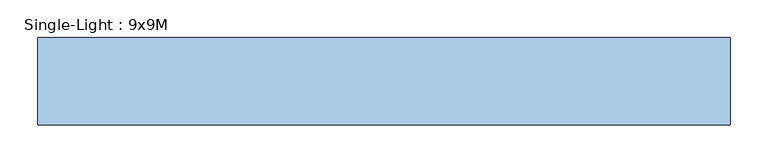
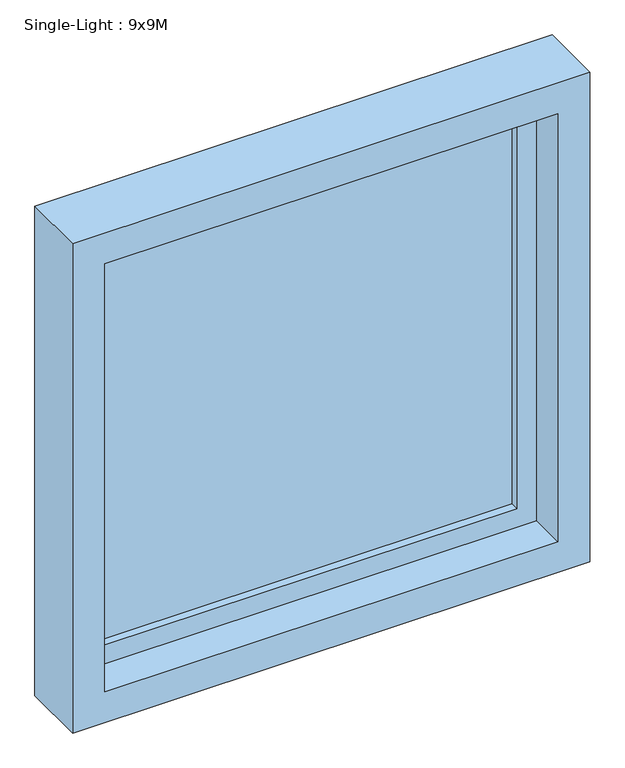
"""IFC4 building model written with IfcOpenShell, lengths in millimetres: window geometry, Single-Light : 9x9M."""

import ifcopenshell
import ifcopenshell.guid

model = None  # the IFC model being written
_history = None  # IfcOwnerHistory: only IFC2X3 demands one
_inside = {}  # id of a spatial element -> (the spatial element, [elements in it])
_under = {}  # id of a project, library or spatial element -> (it, [spatial elements below it])
_declared = {}  # id of a project -> (the project, [libraries it declares])
_typed = {}  # id of a type object -> (the type object, [elements of that type])
_made_of = {}  # id of a material, layer set ... -> (it, [elements and type objects made of it])


def new_model(schema):
    """Start an empty IFC model of exactly this schema.

    Asked for "IFC4X3", IfcOpenShell would pick the latest addendum, in which some entities
    have other attributes; the version numbers below select the first issue.
    IFC2X3 requires an IfcOwnerHistory on every rooted entity: one is made here for all.
    """
    global model, _history
    if schema == "IFC4X3":
        model = ifcopenshell.file(schema_version=(4, 3, 0, 0))
    else:
        model = ifcopenshell.file(schema=schema)
    _inside.clear()
    _under.clear()
    _declared.clear()
    _typed.clear()
    _made_of.clear()
    _history = None
    if model.schema == "IFC2X3":
        org = make("IfcOrganization", Name="unknown")
        user = make(
            "IfcPersonAndOrganization",
            ThePerson=make("IfcPerson", FamilyName="unknown"),
            TheOrganization=org,
        )
        app = make(
            "IfcApplication",
            ApplicationDeveloper=org,
            Version="unknown",
            ApplicationFullName="unknown",
            ApplicationIdentifier="unknown",
        )
        _history = make(
            "IfcOwnerHistory",
            OwningUser=user,
            OwningApplication=app,
            ChangeAction="ADDED",
            CreationDate=0,
        )
    return model


def make(cls, **values):
    """One entity of the class cls with the attributes given. An attribute that is None is left unset."""
    return model.create_entity(
        cls, **{name: value for name, value in values.items() if value is not None}
    )


def rooted(cls, **values):
    """An entity with a GlobalId (a new one), such as an element, a storey or a relation."""
    return make(cls, GlobalId=ifcopenshell.guid.new(), OwnerHistory=_history, **values)


def si_unit(unit_type, name, prefix=None):
    """IfcSIUnit, for example si_unit("LENGTHUNIT", "METRE", prefix="MILLI")."""
    return make("IfcSIUnit", UnitType=unit_type, Prefix=prefix, Name=name)


def assignment(units):
    """IfcUnitAssignment: the units of a project."""
    return None if units is None else make("IfcUnitAssignment", Units=units)


def point(xyz):
    """IfcCartesianPoint."""
    return None if xyz is None else make("IfcCartesianPoint", Coordinates=xyz)


def direction(xyz):
    """IfcDirection."""
    return None if xyz is None else make("IfcDirection", DirectionRatios=xyz)


def frame(location, z_axis=None, x_axis=None):
    """IfcAxis2Placement3D, a coordinate frame: its origin and axes. An axis left out is left unset."""
    return make(
        "IfcAxis2Placement3D",
        Location=point(location),
        Axis=direction(z_axis),
        RefDirection=direction(x_axis),
    )


def origin():
    """The frame at (0, 0, 0) with its axes left unset."""
    return frame((0.0, 0.0, 0.0))


def place(relative_to, where):
    """IfcLocalPlacement: puts the frame where relative to a parent placement (None: the world)."""
    return make(
        "IfcLocalPlacement", PlacementRelTo=relative_to, RelativePlacement=where
    )


def context(
    kind, dimensions, precision=None, world=None, true_north=None, identifier=None
):
    """IfcGeometricRepresentationContext, for example the 3D "Model" context."""
    return make(
        "IfcGeometricRepresentationContext",
        ContextIdentifier=identifier,
        ContextType=kind,
        CoordinateSpaceDimension=dimensions,
        Precision=precision,
        WorldCoordinateSystem=world,
        TrueNorth=true_north,
    )


def project(units=None, contexts=None):
    """IfcProject with its units and contexts."""
    return rooted(
        "IfcProject",
        Name="project",
        RepresentationContexts=contexts,
        UnitsInContext=assignment(units),
    )


def spatial(cls, under=None, at=None, **own):
    """A site, building, storey or space (cls), placed at a placement, below another one or the project."""
    s = rooted(cls, ObjectPlacement=at, **own)
    if under is not None:
        _under.setdefault(under.id(), (under, []))[1].append(s)
    return s


def polyline(points):
    """IfcPolyline through the points."""
    return make("IfcPolyline", Points=[point(p) for p in points])


def outline(outer, holes=None, kind="AREA"):
    """IfcArbitraryClosedProfileDef: a profile drawn as a closed curve; with holes, ...WithVoids."""
    if holes is None:
        return make("IfcArbitraryClosedProfileDef", ProfileType=kind, OuterCurve=outer)
    return make(
        "IfcArbitraryProfileDefWithVoids",
        ProfileType=kind,
        OuterCurve=outer,
        InnerCurves=holes,
    )


def extrude(swept, where, along, depth):
    """IfcExtrudedAreaSolid: the profile swept, set in the frame where, extruded along a direction by depth."""
    return make(
        "IfcExtrudedAreaSolid",
        SweptArea=swept,
        Position=where,
        ExtrudedDirection=direction(along),
        Depth=depth,
    )


def faces_of(points, faces, orient=None, outer=None):
    """IfcFace entities. A face is a list of loops; a loop is a list of indices into points, from 0.

    orient and outer hold one flag for each loop. By default every Orientation is true, the
    first loop of a face is its IfcFaceOuterBound and the others are IfcFaceBound.
    """
    made = []
    for i, loops in enumerate(faces):
        bounds = []
        for j, loop in enumerate(loops):
            is_outer = j == 0 if outer is None else outer[i][j]
            bounds.append(
                make(
                    "IfcFaceOuterBound" if is_outer else "IfcFaceBound",
                    Bound=make("IfcPolyLoop", Polygon=[points[k] for k in loop]),
                    Orientation=True if orient is None else orient[i][j],
                )
            )
        made.append(make("IfcFace", Bounds=bounds))
    return made


def faceted_brep(points, faces, orient=None, outer=None, voids=None):
    """IfcFacetedBrep: a solid bounded by flat faces; with voids (closed shells), ...WithVoids."""
    shared = [point(p) for p in points]
    hull = make("IfcClosedShell", CfsFaces=faces_of(shared, faces, orient, outer))
    if voids is None:
        return make("IfcFacetedBrep", Outer=hull)
    return make(
        "IfcFacetedBrepWithVoids",
        Outer=hull,
        Voids=[
            make(cls, CfsFaces=faces_of(shared, fs, o, b)) for cls, fs, o, b in voids
        ],
    )


def shape(context_of_items, identifier, shape_type, items):
    """IfcShapeRepresentation: the items that make up one representation, for example the "Body"."""
    return make(
        "IfcShapeRepresentation",
        ContextOfItems=context_of_items,
        RepresentationIdentifier=identifier,
        RepresentationType=shape_type,
        Items=items,
    )


def source(mapping_origin, context_of_items, identifier, shape_type, items):
    """IfcRepresentationMap: a shape defined once, which mapped items show again and again."""
    return make(
        "IfcRepresentationMap",
        MappingOrigin=mapping_origin,
        MappedRepresentation=shape(context_of_items, identifier, shape_type, items),
    )


def transform(
    local_origin,
    x_axis=None,
    y_axis=None,
    z_axis=None,
    scale=None,
    scale2=None,
    scale3=None,
    uniform=True,
):
    """IfcCartesianTransformationOperator3D, or its non-uniform kind. x_axis, y_axis, z_axis: its Axis1, 2, 3."""
    if uniform:
        return make(
            "IfcCartesianTransformationOperator3D",
            Axis1=direction(x_axis),
            Axis2=direction(y_axis),
            LocalOrigin=point(local_origin),
            Scale=scale,
            Axis3=direction(z_axis),
        )
    return make(
        "IfcCartesianTransformationOperator3DnonUniform",
        Axis1=direction(x_axis),
        Axis2=direction(y_axis),
        LocalOrigin=point(local_origin),
        Scale=scale,
        Axis3=direction(z_axis),
        Scale2=scale2,
        Scale3=scale3,
    )


def mapped(mapping_source, mapping_target):
    """IfcMappedItem: shows the shape of a source again, moved by a transform."""
    return make(
        "IfcMappedItem", MappingSource=mapping_source, MappingTarget=mapping_target
    )


def made_of(thing, what):
    """Note that an element or type object is made of a material, layer set ...; save() writes the relation."""
    if what is not None:
        _made_of.setdefault(what.id(), (what, []))[1].append(thing)
    return thing


def element(
    cls,
    number,
    at=None,
    inside=None,
    cuts=None,
    type_object=None,
    material=None,
    context=None,
    identifier="Body",
    shape_type=None,
    held_by="IfcProductDefinitionShape",
    body=None,
    shapes=None,
    **own,
):
    """One element of the class cls, such as IfcWall. Its Tag is "e" and its number.

    at: its placement. inside: the storey or other place that contains it. cuts: it is an
    opening in that element (IfcRelVoidsElement). A single representation is given by context,
    identifier, shape_type and body (its items); several are given by shapes. held_by: the class
    of the entity that holds the representations. save() writes the other relations.
    """
    e = rooted(cls, Tag="e%d" % number, ObjectPlacement=at, **own)
    if body is not None:
        shapes = [shape(context, identifier, shape_type, body)]
    if shapes is not None:
        e.Representation = make(held_by, Representations=shapes)
    if inside is not None:
        _inside.setdefault(inside.id(), (inside, []))[1].append(e)
    if cuts is not None:
        rooted(
            "IfcRelVoidsElement", RelatingBuildingElement=cuts, RelatedOpeningElement=e
        )
    if type_object is not None:
        _typed.setdefault(type_object.id(), (type_object, []))[1].append(e)
    return made_of(e, material)


def aggregate(whole, parts):
    """IfcRelAggregates: a whole, such as a stair, and the parts it consists of."""
    return rooted("IfcRelAggregates", RelatingObject=whole, RelatedObjects=parts)


def save(model, path):
    """Write the relations noted so far, then the file.

    IfcRelAggregates (storeys below a building ...), IfcRelContainedInSpatialStructure (elements
    in a storey), IfcRelDefinesByType, IfcRelAssociatesMaterial and IfcRelDeclares: one each for
    every whole, place, type object, material and project.
    """
    for whole, parts in _under.values():
        aggregate(whole, parts)
    for where, things in _inside.values():
        rooted(
            "IfcRelContainedInSpatialStructure",
            RelatedElements=things,
            RelatingStructure=where,
        )
    for kind, things in _typed.values():
        rooted("IfcRelDefinesByType", RelatedObjects=things, RelatingType=kind)
    for what, things in _made_of.values():
        rooted("IfcRelAssociatesMaterial", RelatedObjects=things, RelatingMaterial=what)
    for by, libraries in _declared.values():
        rooted("IfcRelDeclares", RelatingContext=by, RelatedDefinitions=libraries)
    model.write(path)


def single_light_9x9m_9d4aa27d(model_context):
    return source(origin(), model_context, "Body", "SolidModel", [
        extrude(outline(polyline([(1670.0, -414.0), (842.0, -414.0), (842.0, 414.0), (1670.0, 414.0), (1670.0, -414.0)]), holes=[polyline([(1620.0, 364.0), (892.0, 364.0), (892.0, -364.0), (1620.0, -364.0), (1620.0, 364.0)])]), frame((0.0, 134.0, 0.0), z_axis=(0.0, 1.0, 0.0), x_axis=(0.0, 0.0, 1.0)), (0.0, 0.0, 1.0), 50.0),
        faceted_brep([(-456.0, 69.0, 800.0), (-456.0, 184.0, 800.0), (456.0, 184.0, 800.0), (456.0, 69.0, 800.0), (456.0, 184.0, 1712.0), (456.0, 69.0, 1712.0), (-456.0, 184.0, 1712.0), (414.0, 184.0, 1670.0), (-414.0, 184.0, 1670.0), (-414.0, 184.0, 842.0), (414.0, 184.0, 842.0), (-456.0, 69.0, 1712.0), (399.0, 69.0, 857.0), (-399.0, 69.0, 857.0), (-399.0, 69.0, 1655.0), (399.0, 69.0, 1655.0), (-399.0, 134.0, 857.0), (399.0, 134.0, 857.0), (399.0, 134.0, 1655.0), (414.0, 134.0, 842.0), (-414.0, 134.0, 842.0), (-414.0, 134.0, 1670.0), (414.0, 134.0, 1670.0), (-399.0, 134.0, 1655.0)], [[[0, 1, 2, 3]], [[3, 2, 4, 5]], [[2, 1, 6, 4], [7, 8, 9, 10]], [[5, 11, 0, 3], [12, 13, 14, 15]], [[16, 13, 12, 17]], [[17, 12, 15, 18]], [[19, 20, 21, 22], [18, 23, 16, 17]], [[9, 20, 19, 10]], [[10, 19, 22, 7]], [[11, 6, 1, 0]], [[23, 14, 13, 16]], [[8, 21, 20, 9]], [[5, 4, 6, 11]], [[18, 15, 14, 23]], [[7, 22, 21, 8]]]),
        extrude(outline(polyline([(-364.0, 170.0), (364.0, 170.0), (364.0, 148.0), (-364.0, 148.0), (-364.0, 170.0)])), frame((0.0, 0.0, 892.0), z_axis=(0.0, 0.0, 1.0), x_axis=(1.0, 0.0, 0.0)), (0.0, 0.0, 1.0), 728.0),
    ])


if __name__ == "__main__":
    model = new_model("IFC4")
    model_context = context("Model", 3, world=origin())
    ifc_project = project(units=[si_unit("LENGTHUNIT", "METRE", prefix="MILLI")], contexts=[model_context])
    site = spatial("IfcSite", under=ifc_project)
    building = spatial("IfcBuilding", under=site)
    placement = place(None, origin())
    single_light_9x9m_shape = single_light_9x9m_9d4aa27d(model_context)
    element("IfcWindow", 1, ObjectType="Single-Light : 9x9M", at=placement, inside=building, context=model_context, shape_type="MappedRepresentation", body=[
        mapped(single_light_9x9m_shape, transform((0.0, 0.0, 0.0), x_axis=(1.0, 0.0, 0.0), y_axis=(0.0, 1.0, 0.0), z_axis=(0.0, 0.0, 1.0))),
    ])
    save(model, "model.ifc")

# Revit data of these elements
# Project information
#   Client Name = "Test Project"
#   Project Address = "Enter address here"
#   Project Number = "Number"
#   Current Version = "0.0.0"
#   SR Document GUID = "3eb9317e-835d-4f79-8926-4d15b96bc824"
# Type "Single-Light : 9x9M"
#   Type Mark = "44"
#   Creator Organization [instance default] = "© Danish Educational Content"
#   Creator Name [instance default] = "© Erik Falck Jørgensen"
#   Creator Build [instance default] = "2017.0801.0"
#   Analytic Construction = "<None>"
#   length#5 = -36 mm
#   length#4 = -14 mm
#   length#3 = 120 mm
#   length#2 = 57 mm
#   length#1 = 0 mm
#   Seal Width = 12 mm
#   Rough Width = 912 mm
#   Rough Height = 912 mm
#   Rebate Depth = 50 mm
#   Rabbet Width = 15 mm
#   Rabbet Depth = 50 mm
#   Height = 888 mm
#   Glass Thickness = 22 mm
#   Frame Width = 50 mm
#   Frame Depth = 50 mm
#   Exterior Direction [instance default] = 0.00°
#   Case Depth = 115 mm
#   Case Width = 45 mm
#   Default Sill Height = 800 mm
#   Width = 888 mm
#   Sealing = no
#   Hinging = yes
#   Wall Closure = 1
#   Above Cutplane [instance default] = no
#   Wall Surface = none
#   Sill Plate = none
#   Glass = none
#   Frame/Mullion = none
#   Embrasure = none
#   Case/Transom = none
# Element 1 (IfcWindow, "Single-Light : 9x9M")
#   Materials on its faces: "Default Frame/Mullion (Interior/Exterior)", "Glass"
# Materials
#   "Default Frame/Mullion (Interior/Exterior)": class "Generic", colour RGB 205 205 205, transparency 0, Description = "Udefineret karm/ramme materiale", Cost = 0
#   "Glass": class "Glass", colour RGB 180 200 255, transparency 0.75, Description = "Generisk glas", Cost = 0
